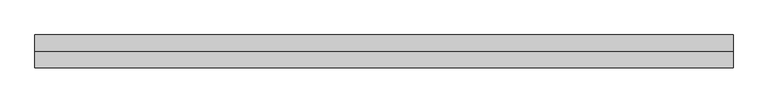
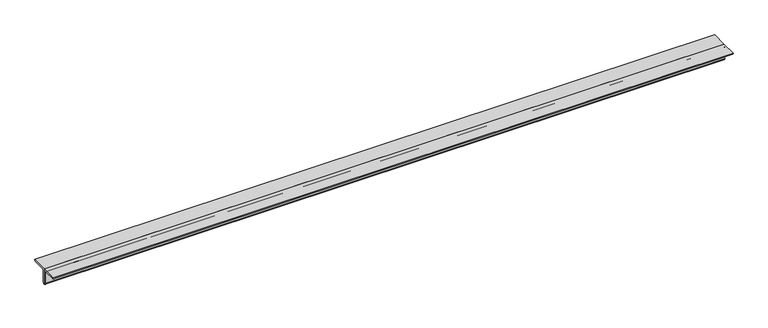
"""IFC4 building model written with IfcOpenShell, lengths in millimetres: member geometry, Steel Framing_2Ls_KS : H_SB_AR_S02_2Ls-100x100x10_VBR1."""

from ifc_helpers import new_model, si_unit, point, frame, frame_2d, origin, place, context, project, spatial, polyline, circle_curve, trimmed, segment, composite_curve, outline, extrude, source, transform, mapped, element, save


def member_33af7571(model_context):
    return source(origin(), model_context, "Body", "SweptSolid", [
        extrude(outline(composite_curve([segment(polyline([(0.0, 28.2), (100.0, 28.2)]), True, "CONTINUOUS"), segment(trimmed(circle_curve(frame_2d((90.0, 28.2)), 10.0), [point((100.0, 28.2))], [point((90.0, 18.2))], False, "CARTESIAN"), True, "CONTINUOUS"), segment(polyline([(90.0, 18.2), (20.0, 18.2)]), True, "CONTINUOUS"), segment(trimmed(circle_curve(frame_2d((20.0, 8.2)), 10.0), [point((20.0, 18.2))], [point((10.0, 8.2))], True, "CARTESIAN"), True, "CONTINUOUS"), segment(polyline([(10.0, 8.2), (10.0, -61.8)]), True, "CONTINUOUS"), segment(trimmed(circle_curve(frame_2d((0.0, -61.8)), 10.0), [point((10.0, -61.8))], [point((0.0, -71.8))], False, "CARTESIAN"), True, "CONTINUOUS"), segment(polyline([(0.0, -71.8), (0.0, 28.2)]), True, "CONTINUOUS")], self_intersect=False)), frame((-2190.4397751, 0.0, 0.0), z_axis=(1.0, 0.0, 0.0), x_axis=(0.0, 1.0, 0.0)), (0.0, 0.0, 1.0), 4232.1149008),
        extrude(outline(composite_curve([segment(polyline([(0.0, 28.2), (0.0, -71.8)]), True, "CONTINUOUS"), segment(trimmed(circle_curve(frame_2d((0.0, -61.8)), 10.0), [point((0.0, -71.8))], [point((-10.0, -61.8))], False, "CARTESIAN"), True, "CONTINUOUS"), segment(polyline([(-10.0, -61.8), (-10.0, 8.2)]), True, "CONTINUOUS"), segment(trimmed(circle_curve(frame_2d((-20.0, 8.2)), 10.0), [point((-10.0, 8.2))], [point((-20.0, 18.2))], True, "CARTESIAN"), True, "CONTINUOUS"), segment(polyline([(-20.0, 18.2), (-90.0, 18.2)]), True, "CONTINUOUS"), segment(trimmed(circle_curve(frame_2d((-90.0, 28.2)), 10.0), [point((-90.0, 18.2))], [point((-100.0, 28.2))], False, "CARTESIAN"), True, "CONTINUOUS"), segment(polyline([(-100.0, 28.2), (0.0, 28.2)]), True, "CONTINUOUS")], self_intersect=False)), frame((-2190.4397751, 0.0, 0.0), z_axis=(1.0, 0.0, 0.0), x_axis=(0.0, 1.0, 0.0)), (0.0, 0.0, 1.0), 4232.1149008),
    ])


if __name__ == "__main__":
    model = new_model("IFC4")
    model_context = context("Model", 3, world=origin())
    ifc_project = project(units=[si_unit("LENGTHUNIT", "METRE", prefix="MILLI")], contexts=[model_context])
    site = spatial("IfcSite", under=ifc_project)
    building = spatial("IfcBuilding", under=site)
    placement = place(None, origin())
    member_shape = member_33af7571(model_context)
    element("IfcMember", 1, ObjectType="Steel Framing_2Ls_KS : H_SB_AR_S02_2Ls-100x100x10_VBR1", at=placement, inside=building, context=model_context, shape_type="MappedRepresentation", body=[
        mapped(member_shape, transform((0.0, 0.0, 0.0), x_axis=(1.0, 0.0, 0.0), y_axis=(0.0, 1.0, 0.0), z_axis=(0.0, 0.0, 1.0))),
    ])
    save(model, "model.ifc")

# Revit data of these elements
# Type "Steel Framing_2Ls_KS : H_SB_AR_S02_2Ls-100x100x10_VBR1"
#   Type Comments = "MAIN"
#   Type Mark = "VBR1"
#   H_SectionID = "2Ls-100x100x10"
#   Assembly Code = "B10"
#   Legs = "LLBB"
#   H_Ratio for Additional Steel Plate = 0.2
#   W = 0
#   Perimeter = 0.80 m²/m
#   Nominal Weight = 29.80 kgf/m
#   Length [instance default] = 1524 mm
#   Space = 0 mm
#   b = 100 mm
#   d = 100 mm
#   t = 10 mm
#   y = 28.2 mm
#   A = 0.0038 m²
#   Structural Material [instance default] = Steel, 45-345
# Element 1 (IfcMember, "Steel Framing_2Ls_KS : H_SB_AR_S02_2Ls-100x100x10_VBR1")
#   Materials on its faces: "Steel, 45-345"
# Materials
#   "Steel, 45-345": class "Metal", colour RGB 189 187 185, transparency 0, Description = "Steel 345 MPa", Cost = 0
